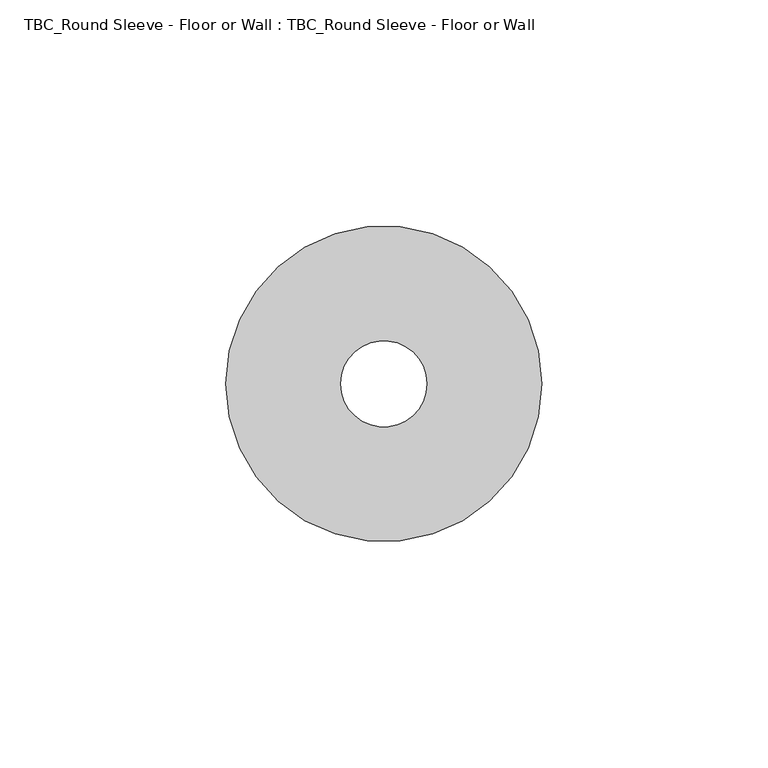
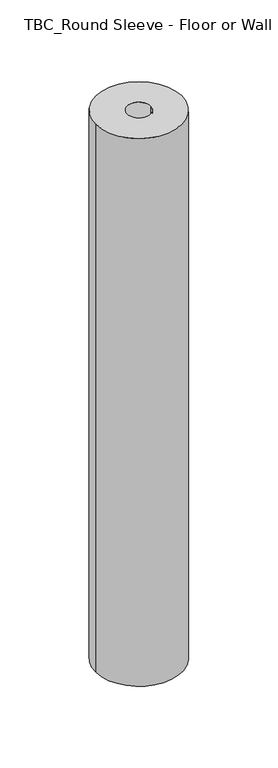
"""IFC4 building model written with IfcOpenShell, lengths in millimetres: proxy geometry, TBC_Round Sleeve - Floor or Wall : TBC_Round Sleeve - Floor or Wall."""

from ifc_helpers import new_model, si_unit, point, frame, origin, origin_2d, place, context, project, spatial, circle_curve, trimmed, segment, composite_curve, outline, extrude, source, transform, mapped, element, save


def tbc_round_sleeve_floor_or_wall_tbc_round_sleeve_floor_or_269cfd1e(model_context):
    return source(origin(), model_context, "Body", "SweptSolid", [
        extrude(outline(composite_curve([segment(trimmed(circle_curve(origin_2d(), 34.925), [point((-34.925, 0.0))], [point((34.925, 0.0))], False, "CARTESIAN"), True, "CONTINUOUS"), segment(trimmed(circle_curve(origin_2d(), 34.925), [point((34.925, 0.0))], [point((-34.925, 0.0))], False, "CARTESIAN"), True, "CONTINUOUS")], self_intersect=False), holes=[composite_curve([segment(trimmed(circle_curve(origin_2d(), 9.525), [point((-9.525, 0.0))], [point((9.525, 0.0))], True, "CARTESIAN"), True, "CONTINUOUS"), segment(trimmed(circle_curve(origin_2d(), 9.525), [point((9.525, 0.0))], [point((-9.525, 0.0))], True, "CARTESIAN"), True, "CONTINUOUS")], self_intersect=False)]), frame((0.0, 0.0, -469.9), z_axis=(0.0, 0.0, 1.0), x_axis=(1.0, 0.0, 0.0)), (0.0, 0.0, 1.0), 469.9),
    ])


if __name__ == "__main__":
    model = new_model("IFC4")
    model_context = context("Model", 3, world=origin())
    ifc_project = project(units=[si_unit("LENGTHUNIT", "METRE", prefix="MILLI")], contexts=[model_context])
    site = spatial("IfcSite", under=ifc_project)
    building = spatial("IfcBuilding", under=site)
    placement = place(None, origin())
    tbc_round_sleeve_floor_or_wall_tbc_round_sleeve_floor_or_shape = tbc_round_sleeve_floor_or_wall_tbc_round_sleeve_floor_or_269cfd1e(model_context)
    element("IfcBuildingElementProxy", 1, Name="TBC_Round Sleeve - Floor or Wall : TBC_Round Sleeve - Floor or Wall", ObjectType="TBC_Round Sleeve - Floor or Wall : TBC_Round Sleeve - Floor or Wall", at=placement, inside=building, context=model_context, shape_type="MappedRepresentation", body=[
        mapped(tbc_round_sleeve_floor_or_wall_tbc_round_sleeve_floor_or_shape, transform((0.0, 0.0, 0.0), x_axis=(1.0, 0.0, 0.0), y_axis=(0.0, 1.0, 0.0), z_axis=(0.0, 0.0, 1.0))),
    ])
    save(model, "model.ifc")

# Revit data of these elements
# Type "TBC_Round Sleeve - Floor or Wall : TBC_Round Sleeve - Floor or Wall"
#   Tag Dimension [instance default] = ""
#   MEP Type [instance default] = ""
#   MEP Element [instance default] = ""
#   MEP Category [instance default] = ""
#   Host Element Type [instance default] = ""
#   Host Element Id [instance default] = ""
#   Host Element Category [instance default] = ""
#   Control Line Y [instance default] = ""
#   Control Line X [instance default] = ""
#   Sleeve Radius [instance default] = 1' - 0"
#   Sleeve Edge [instance default] = 1' - 2"
#   Sleeve Depth [instance default] = 3' - 0"
#   Distance Y [instance default] = 0' - 0"
#   Distance X [instance default] = 0' - 0"
#   Default Elevation = 0
# Element 1 (IfcBuildingElementProxy, "TBC_Round Sleeve - Floor or Wall : TBC_Round Sleeve - Floor or Wall")
#   Sleeve Radius = 0' - 0 3/4"
#   Sleeve Edge = 0' - 2 3/4"
#   Sleeve Depth = 1' - 6 1/2"
